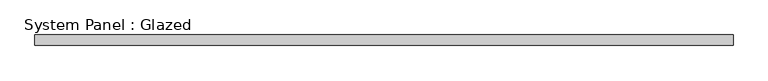
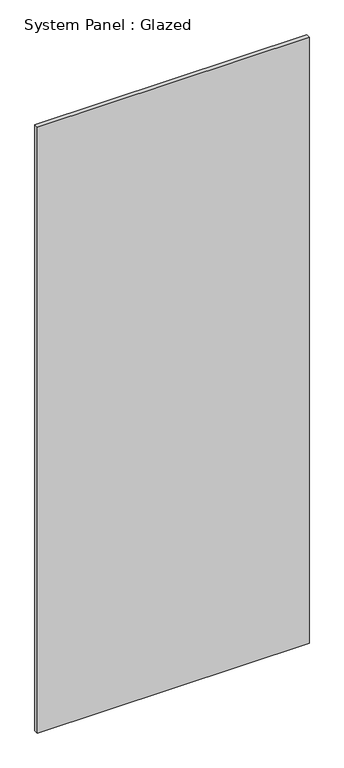
"""IFC4 building model written with IfcOpenShell, lengths in millimetres: plate geometry, System Panel : Glazed."""

from ifc_helpers import new_model, si_unit, origin, origin_with_axes, place, context, project, spatial, polyline, outline, extrude, source, transform, mapped, element, save


def system_panel_glazed_6f64ce2d(model_context):
    return source(origin(), model_context, "Body", "SweptSolid", [
        extrude(outline(polyline([(827.5000002, 24.5), (-827.5000002, 24.5), (-827.5000002, 49.5), (827.5000002, 49.5), (827.5000002, 24.5)])), origin_with_axes(), (0.0, 0.0, 1.0), 3900.0),
    ])


if __name__ == "__main__":
    model = new_model("IFC4")
    model_context = context("Model", 3, world=origin())
    ifc_project = project(units=[si_unit("LENGTHUNIT", "METRE", prefix="MILLI")], contexts=[model_context])
    site = spatial("IfcSite", under=ifc_project)
    building = spatial("IfcBuilding", under=site)
    placement = place(None, origin())
    system_panel_glazed_shape = system_panel_glazed_6f64ce2d(model_context)
    element("IfcPlate", 1, ObjectType="System Panel : Glazed", at=placement, inside=building, context=model_context, shape_type="MappedRepresentation", body=[
        mapped(system_panel_glazed_shape, transform((0.0, 0.0, 0.0), x_axis=(1.0, 0.0, 0.0), y_axis=(0.0, 1.0, 0.0), z_axis=(0.0, 0.0, 1.0))),
    ])
    save(model, "model.ifc")

# Revit data of these elements
# Type "System Panel : Glazed"
#   Keynote = "H11"
#   Construction Type Id = "GSP4R"
#   Analytic Construction = "1/8 in Pilkington single glazing"
#   Visual Light Transmittance = 0.9
#   Solar Heat Gain Coefficient = 0.86
#   Heat Transfer Coefficient (U) = 6.7069 W/(m²·K)
#   Define Thermal Properties by = 1
# Element 1 (IfcPlate, "System Panel : Glazed")
#   Materials on its faces: "Glass"
# Materials
#   "Glass": class "Glass", colour RGB 0 128 192, transparency 0.9, Description = "Soda Lime Glass", Cost = 0
